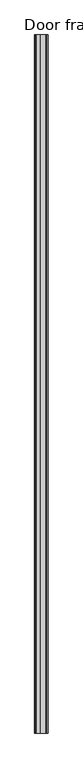
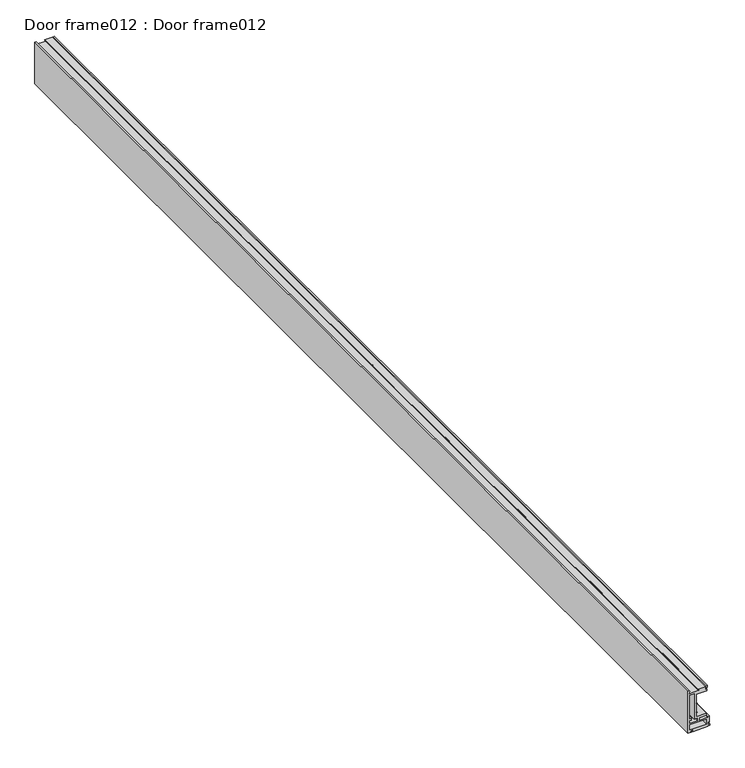
"""IFC4 building model written with IfcOpenShell, lengths in millimetres: proxy geometry, Door frame012 : Door frame012."""

import ifcopenshell
import ifcopenshell.guid

model = None  # the IFC model being written
_history = None  # IfcOwnerHistory: only IFC2X3 demands one
_inside = {}  # id of a spatial element -> (the spatial element, [elements in it])
_under = {}  # id of a project, library or spatial element -> (it, [spatial elements below it])
_declared = {}  # id of a project -> (the project, [libraries it declares])
_typed = {}  # id of a type object -> (the type object, [elements of that type])
_made_of = {}  # id of a material, layer set ... -> (it, [elements and type objects made of it])


def new_model(schema):
    """Start an empty IFC model of exactly this schema.

    Asked for "IFC4X3", IfcOpenShell would pick the latest addendum, in which some entities
    have other attributes; the version numbers below select the first issue.
    IFC2X3 requires an IfcOwnerHistory on every rooted entity: one is made here for all.
    """
    global model, _history
    if schema == "IFC4X3":
        model = ifcopenshell.file(schema_version=(4, 3, 0, 0))
    else:
        model = ifcopenshell.file(schema=schema)
    _inside.clear()
    _under.clear()
    _declared.clear()
    _typed.clear()
    _made_of.clear()
    _history = None
    if model.schema == "IFC2X3":
        org = make("IfcOrganization", Name="unknown")
        user = make(
            "IfcPersonAndOrganization",
            ThePerson=make("IfcPerson", FamilyName="unknown"),
            TheOrganization=org,
        )
        app = make(
            "IfcApplication",
            ApplicationDeveloper=org,
            Version="unknown",
            ApplicationFullName="unknown",
            ApplicationIdentifier="unknown",
        )
        _history = make(
            "IfcOwnerHistory",
            OwningUser=user,
            OwningApplication=app,
            ChangeAction="ADDED",
            CreationDate=0,
        )
    return model


def make(cls, **values):
    """One entity of the class cls with the attributes given. An attribute that is None is left unset."""
    return model.create_entity(
        cls, **{name: value for name, value in values.items() if value is not None}
    )


def rooted(cls, **values):
    """An entity with a GlobalId (a new one), such as an element, a storey or a relation."""
    return make(cls, GlobalId=ifcopenshell.guid.new(), OwnerHistory=_history, **values)


def si_unit(unit_type, name, prefix=None):
    """IfcSIUnit, for example si_unit("LENGTHUNIT", "METRE", prefix="MILLI")."""
    return make("IfcSIUnit", UnitType=unit_type, Prefix=prefix, Name=name)


def assignment(units):
    """IfcUnitAssignment: the units of a project."""
    return None if units is None else make("IfcUnitAssignment", Units=units)


def point(xyz):
    """IfcCartesianPoint."""
    return None if xyz is None else make("IfcCartesianPoint", Coordinates=xyz)


def direction(xyz):
    """IfcDirection."""
    return None if xyz is None else make("IfcDirection", DirectionRatios=xyz)


def frame(location, z_axis=None, x_axis=None):
    """IfcAxis2Placement3D, a coordinate frame: its origin and axes. An axis left out is left unset."""
    return make(
        "IfcAxis2Placement3D",
        Location=point(location),
        Axis=direction(z_axis),
        RefDirection=direction(x_axis),
    )


def origin():
    """The frame at (0, 0, 0) with its axes left unset."""
    return frame((0.0, 0.0, 0.0))


def place(relative_to, where):
    """IfcLocalPlacement: puts the frame where relative to a parent placement (None: the world)."""
    return make(
        "IfcLocalPlacement", PlacementRelTo=relative_to, RelativePlacement=where
    )


def context(
    kind, dimensions, precision=None, world=None, true_north=None, identifier=None
):
    """IfcGeometricRepresentationContext, for example the 3D "Model" context."""
    return make(
        "IfcGeometricRepresentationContext",
        ContextIdentifier=identifier,
        ContextType=kind,
        CoordinateSpaceDimension=dimensions,
        Precision=precision,
        WorldCoordinateSystem=world,
        TrueNorth=true_north,
    )


def project(units=None, contexts=None):
    """IfcProject with its units and contexts."""
    return rooted(
        "IfcProject",
        Name="project",
        RepresentationContexts=contexts,
        UnitsInContext=assignment(units),
    )


def spatial(cls, under=None, at=None, **own):
    """A site, building, storey or space (cls), placed at a placement, below another one or the project."""
    s = rooted(cls, ObjectPlacement=at, **own)
    if under is not None:
        _under.setdefault(under.id(), (under, []))[1].append(s)
    return s


def polyline(points):
    """IfcPolyline through the points."""
    return make("IfcPolyline", Points=[point(p) for p in points])


def outline(outer, holes=None, kind="AREA"):
    """IfcArbitraryClosedProfileDef: a profile drawn as a closed curve; with holes, ...WithVoids."""
    if holes is None:
        return make("IfcArbitraryClosedProfileDef", ProfileType=kind, OuterCurve=outer)
    return make(
        "IfcArbitraryProfileDefWithVoids",
        ProfileType=kind,
        OuterCurve=outer,
        InnerCurves=holes,
    )


def extrude(swept, where, along, depth):
    """IfcExtrudedAreaSolid: the profile swept, set in the frame where, extruded along a direction by depth."""
    return make(
        "IfcExtrudedAreaSolid",
        SweptArea=swept,
        Position=where,
        ExtrudedDirection=direction(along),
        Depth=depth,
    )


def shape(context_of_items, identifier, shape_type, items):
    """IfcShapeRepresentation: the items that make up one representation, for example the "Body"."""
    return make(
        "IfcShapeRepresentation",
        ContextOfItems=context_of_items,
        RepresentationIdentifier=identifier,
        RepresentationType=shape_type,
        Items=items,
    )


def source(mapping_origin, context_of_items, identifier, shape_type, items):
    """IfcRepresentationMap: a shape defined once, which mapped items show again and again."""
    return make(
        "IfcRepresentationMap",
        MappingOrigin=mapping_origin,
        MappedRepresentation=shape(context_of_items, identifier, shape_type, items),
    )


def transform(
    local_origin,
    x_axis=None,
    y_axis=None,
    z_axis=None,
    scale=None,
    scale2=None,
    scale3=None,
    uniform=True,
):
    """IfcCartesianTransformationOperator3D, or its non-uniform kind. x_axis, y_axis, z_axis: its Axis1, 2, 3."""
    if uniform:
        return make(
            "IfcCartesianTransformationOperator3D",
            Axis1=direction(x_axis),
            Axis2=direction(y_axis),
            LocalOrigin=point(local_origin),
            Scale=scale,
            Axis3=direction(z_axis),
        )
    return make(
        "IfcCartesianTransformationOperator3DnonUniform",
        Axis1=direction(x_axis),
        Axis2=direction(y_axis),
        LocalOrigin=point(local_origin),
        Scale=scale,
        Axis3=direction(z_axis),
        Scale2=scale2,
        Scale3=scale3,
    )


def mapped(mapping_source, mapping_target):
    """IfcMappedItem: shows the shape of a source again, moved by a transform."""
    return make(
        "IfcMappedItem", MappingSource=mapping_source, MappingTarget=mapping_target
    )


def made_of(thing, what):
    """Note that an element or type object is made of a material, layer set ...; save() writes the relation."""
    if what is not None:
        _made_of.setdefault(what.id(), (what, []))[1].append(thing)
    return thing


def element(
    cls,
    number,
    at=None,
    inside=None,
    cuts=None,
    type_object=None,
    material=None,
    context=None,
    identifier="Body",
    shape_type=None,
    held_by="IfcProductDefinitionShape",
    body=None,
    shapes=None,
    **own,
):
    """One element of the class cls, such as IfcWall. Its Tag is "e" and its number.

    at: its placement. inside: the storey or other place that contains it. cuts: it is an
    opening in that element (IfcRelVoidsElement). A single representation is given by context,
    identifier, shape_type and body (its items); several are given by shapes. held_by: the class
    of the entity that holds the representations. save() writes the other relations.
    """
    e = rooted(cls, Tag="e%d" % number, ObjectPlacement=at, **own)
    if body is not None:
        shapes = [shape(context, identifier, shape_type, body)]
    if shapes is not None:
        e.Representation = make(held_by, Representations=shapes)
    if inside is not None:
        _inside.setdefault(inside.id(), (inside, []))[1].append(e)
    if cuts is not None:
        rooted(
            "IfcRelVoidsElement", RelatingBuildingElement=cuts, RelatedOpeningElement=e
        )
    if type_object is not None:
        _typed.setdefault(type_object.id(), (type_object, []))[1].append(e)
    return made_of(e, material)


def aggregate(whole, parts):
    """IfcRelAggregates: a whole, such as a stair, and the parts it consists of."""
    return rooted("IfcRelAggregates", RelatingObject=whole, RelatedObjects=parts)


def save(model, path):
    """Write the relations noted so far, then the file.

    IfcRelAggregates (storeys below a building ...), IfcRelContainedInSpatialStructure (elements
    in a storey), IfcRelDefinesByType, IfcRelAssociatesMaterial and IfcRelDeclares: one each for
    every whole, place, type object, material and project.
    """
    for whole, parts in _under.values():
        aggregate(whole, parts)
    for where, things in _inside.values():
        rooted(
            "IfcRelContainedInSpatialStructure",
            RelatedElements=things,
            RelatingStructure=where,
        )
    for kind, things in _typed.values():
        rooted("IfcRelDefinesByType", RelatedObjects=things, RelatingType=kind)
    for what, things in _made_of.values():
        rooted("IfcRelAssociatesMaterial", RelatedObjects=things, RelatingMaterial=what)
    for by, libraries in _declared.values():
        rooted("IfcRelDeclares", RelatingContext=by, RelatedDefinitions=libraries)
    model.write(path)


def door_frame012_door_frame012_2ed3f318(model_context):
    return source(origin(), model_context, "Body", "SweptSolid", [
        extrude(outline(polyline([(36608.9977225, 15539.5084948), (36608.9977225, 15524.517453), (36613.8237225, 15524.517453), (36613.8237225, 15537.3384133), (36616.9987225, 15537.3384133), (36616.9987225, 15519.5076168), (36623.9157731, 15519.5076168), (36624.8727225, 15520.9106887), (36625.8290531, 15519.5076168), (36640.6803935, 15519.5076168), (36641.6367241, 15520.9106887), (36642.5936735, 15519.5076168), (36658.8030324, 15519.5076168), (36658.8030324, 15538.2476818), (36662.4618113, 15538.2476818), (36661.0188583, 15535.7484139), (36666.3421883, 15535.7484139), (36665.4690732, 15539.0049628), (36668.703989, 15539.288472), (36667.561659, 15536.9486127), (36667.7957063, 15535.7484139), (36667.7957063, 15522.1352688), (36666.5824658, 15522.1352688), (36666.5824658, 15523.6520602), (36664.6229889, 15523.6520602), (36664.6229889, 15506.8580308), (36666.7222221, 15506.8580308), (36668.7089205, 15508.0054504), (36669.4492947, 15507.5857589), (36669.4492947, 15504.8264133), (36591.6236909, 15504.8264133), (36591.6236909, 15510.4085802), (36592.8950628, 15510.4085802), (36592.8950628, 15509.5254133), (36594.1652793, 15509.5254133), (36594.1652793, 15514.0974128), (36592.8950628, 15514.0974128), (36592.8950628, 15513.2142459), (36591.6240434, 15513.2142459), (36591.6240434, 15540.1828722), (36593.5561506, 15540.1828722), (36593.5561506, 15541.3652071), (36592.4137824, 15543.7050664), (36595.6486981, 15543.4215572), (36594.775583, 15540.1650084), (36600.1211436, 15540.1650084), (36598.5843732, 15542.6834949), (36610.4200435, 15542.6834949), (36610.4200435, 15539.5084948), (36608.9977225, 15539.5084948)]), holes=[polyline([(36608.9977225, 15508.0061443), (36613.8237225, 15508.0061443), (36613.8237225, 15511.1764133), (36616.9987225, 15511.1764133), (36616.9987225, 15508.0014133), (36661.4479889, 15508.0014133), (36661.4479889, 15516.3326168), (36613.8237225, 15516.3326168), (36613.8237225, 15521.3411443), (36608.9977225, 15521.3411443), (36608.9977225, 15508.0061443)]), polyline([(36605.8183749, 15537.6432186), (36596.3988909, 15537.6432186), (36596.3988909, 15508.0014133), (36605.8183749, 15508.0014133), (36605.8183749, 15537.6432186)])]), frame((0.0, -1052.8906567, 0.0), z_axis=(0.0, 1.0, 0.0), x_axis=(0.0, 0.0, 1.0)), (0.0, 0.0, 1.0), 1999.85),
    ])


if __name__ == "__main__":
    model = new_model("IFC4")
    model_context = context("Model", 3, world=origin())
    ifc_project = project(units=[si_unit("LENGTHUNIT", "METRE", prefix="MILLI")], contexts=[model_context])
    site = spatial("IfcSite", under=ifc_project)
    building = spatial("IfcBuilding", under=site)
    placement = place(None, origin())
    door_frame012_door_frame012_shape = door_frame012_door_frame012_2ed3f318(model_context)
    element("IfcBuildingElementProxy", 1, Name="Door frame012 : Door frame012", ObjectType="Door frame012 : Door frame012", at=placement, inside=building, context=model_context, shape_type="MappedRepresentation", body=[
        mapped(door_frame012_door_frame012_shape, transform((0.0, 0.0, 0.0), x_axis=(1.0, 0.0, 0.0), y_axis=(0.0, 1.0, 0.0), z_axis=(0.0, 0.0, 1.0))),
    ])
    save(model, "model.ifc")

# Revit data of these elements
# Type "Door frame012 : Door frame012"
#   NameOverride = "Door frame012"
# Element 1 (IfcBuildingElementProxy, "Door frame012 : Door frame012")
#   Materials on its faces: "FLEETWOOD SERIES T-3200 SINGLE SWING DOOR FRAME"
# Materials
#   "FLEETWOOD SERIES T-3200 SINGLE SWING DOOR FRAME": class "Unassigned", colour RGB 128 128 128, transparency 0, Cost = 0
